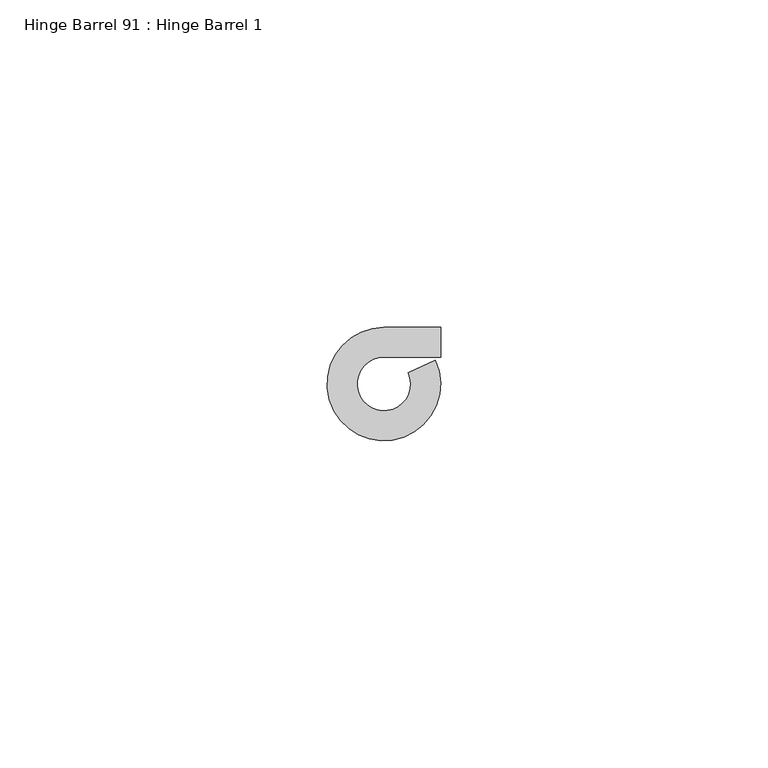
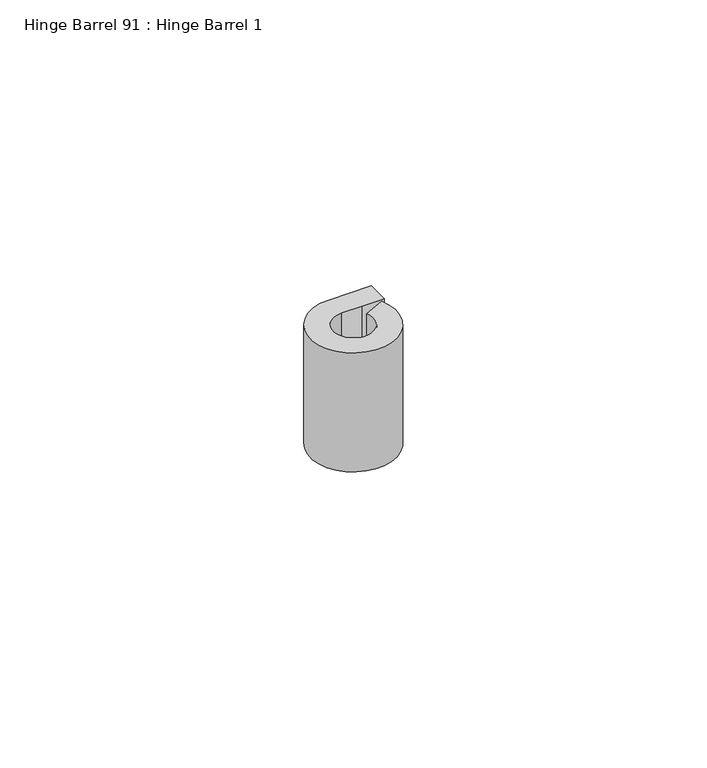
"""IFC4 building model written with IfcOpenShell, lengths in millimetres: proxy geometry, Hinge Barrel 91 : Hinge Barrel 1."""

from ifc_helpers import new_model, si_unit, point, frame, frame_2d, origin, place, context, project, spatial, polyline, circle_curve, trimmed, segment, composite_curve, outline, extrude, source, transform, mapped, element, save


def hinge_barrel_91_hinge_barrel_1_feeece1f(model_context):
    return source(origin(), model_context, "Body", "SweptSolid", [
        extrude(outline(composite_curve([segment(polyline([(587323.2214739, -533980.5883841), (587319.1320739, -533980.5883841)]), True, "CONTINUOUS"), segment(trimmed(circle_curve(frame_2d((587319.1320739, -533984.6777841)), 4.0894), [point((587319.1320739, -533980.5883841))], [point((587322.8436736, -533982.9610371))], True, "CARTESIAN"), True, "CONTINUOUS"), segment(polyline([(587322.8436736, -533982.9610371), (587326.986084, -533981.0450249)]), True, "CONTINUOUS"), segment(trimmed(circle_curve(frame_2d((587319.1320739, -533984.6777841)), 8.6534625), [point((587326.986084, -533981.0450249))], [point((587319.1320739, -533976.0243216))], False, "CARTESIAN"), True, "CONTINUOUS"), segment(polyline([(587319.1320739, -533976.0243216), (587327.7934739, -533976.0243216), (587327.7934739, -533980.5883841), (587323.2214739, -533980.5883841)]), True, "CONTINUOUS")], self_intersect=False)), frame((0.0, 0.0, 311.15), z_axis=(0.0, 0.0, 1.0), x_axis=(1.0, 0.0, 0.0)), (0.0, 0.0, 1.0), 25.4),
    ])


if __name__ == "__main__":
    model = new_model("IFC4")
    model_context = context("Model", 3, world=origin())
    ifc_project = project(units=[si_unit("LENGTHUNIT", "METRE", prefix="MILLI")], contexts=[model_context])
    site = spatial("IfcSite", under=ifc_project)
    building = spatial("IfcBuilding", under=site)
    placement = place(None, origin())
    hinge_barrel_91_hinge_barrel_1_shape = hinge_barrel_91_hinge_barrel_1_feeece1f(model_context)
    element("IfcBuildingElementProxy", 1, Name="Hinge Barrel 91 : Hinge Barrel 1", ObjectType="Hinge Barrel 91 : Hinge Barrel 1", at=placement, inside=building, context=model_context, shape_type="MappedRepresentation", body=[
        mapped(hinge_barrel_91_hinge_barrel_1_shape, transform((0.0, 0.0, 0.0), x_axis=(1.0, 0.0, 0.0), y_axis=(0.0, 1.0, 0.0), z_axis=(0.0, 0.0, 1.0))),
    ])
    save(model, "model.ifc")

# Revit data of these elements
# Element 1 (IfcBuildingElementProxy, "Hinge Barrel 91 : Hinge Barrel 1")
#   Materials on its faces: "6\"X6\" WELD-ON STL BUTT HINGE"
# Materials
#   "6\"X6\" WELD-ON STL BUTT HINGE": class "Metal", colour RGB 189 187 185, transparency 0, Description = "Carbon steel", Cost = 0
